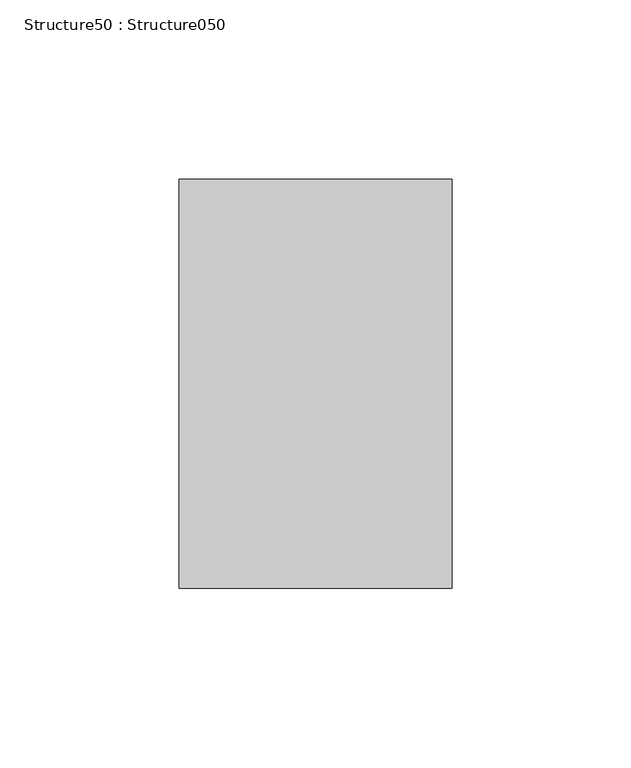
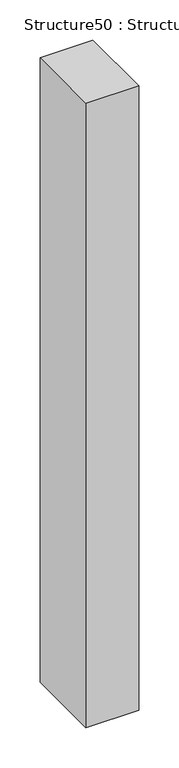
"""IFC4 building model written with IfcOpenShell, lengths in millimetres: proxy geometry, Structure50 : Structure050."""

from ifc_helpers import new_model, si_unit, frame, origin, place, context, project, spatial, polyline, outline, extrude, source, transform, mapped, element, save


def structure50_structure050_92f2a138(model_context):
    return source(origin(), model_context, "Body", "SweptSolid", [
        extrude(outline(polyline([(-38518.0176606, 250877.2787557), (-38518.0176606, 250763.0426193), (-38594.2176606, 250763.0426193), (-38594.2176606, 250877.2787557), (-38518.0176606, 250877.2787557)])), frame((0.0, 0.0, 3528.5825142), z_axis=(0.0, 0.0, 1.0), x_axis=(1.0, 0.0, 0.0)), (0.0, 0.0, 1.0), 951.8594804),
    ])


if __name__ == "__main__":
    model = new_model("IFC4")
    model_context = context("Model", 3, world=origin())
    ifc_project = project(units=[si_unit("LENGTHUNIT", "METRE", prefix="MILLI")], contexts=[model_context])
    site = spatial("IfcSite", under=ifc_project)
    building = spatial("IfcBuilding", under=site)
    placement = place(None, origin())
    structure50_structure050_shape = structure50_structure050_92f2a138(model_context)
    element("IfcBuildingElementProxy", 1, Name="Structure50 : Structure050", ObjectType="Structure50 : Structure050", at=placement, inside=building, context=model_context, shape_type="MappedRepresentation", body=[
        mapped(structure50_structure050_shape, transform((0.0, 0.0, 0.0), x_axis=(1.0, 0.0, 0.0), y_axis=(0.0, 1.0, 0.0), z_axis=(0.0, 0.0, 1.0))),
    ])
    save(model, "model.ifc")

# Revit data of these elements
# Type "Structure50 : Structure050"
#   NameOverride = "Structure050"
# Element 1 (IfcBuildingElementProxy, "Structure50 : Structure050")
#   Materials on its faces: "BRUSHED ALUM. LETTERING"
# Materials
#   "BRUSHED ALUM. LETTERING": class "Unassigned", colour RGB 169 181 186, transparency 0, Cost = 0
